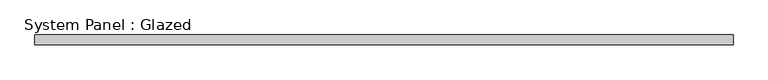
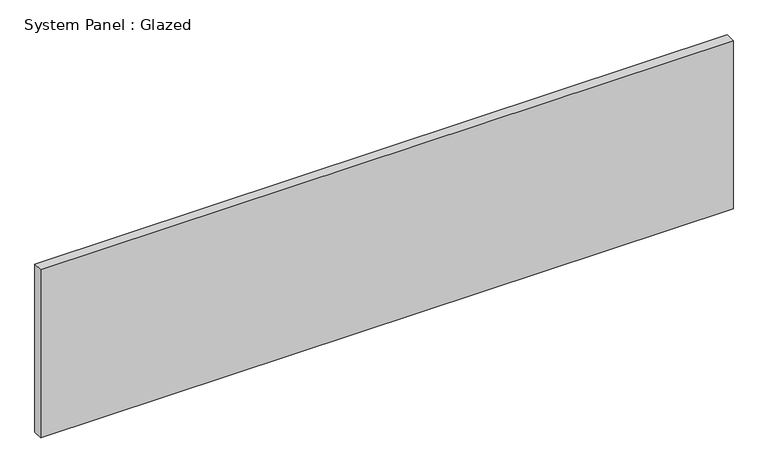
"""IFC4 building model written with IfcOpenShell, lengths in millimetres: plate geometry, System Panel : Glazed."""

import ifcopenshell
import ifcopenshell.guid

model = None  # the IFC model being written
_history = None  # IfcOwnerHistory: only IFC2X3 demands one
_inside = {}  # id of a spatial element -> (the spatial element, [elements in it])
_under = {}  # id of a project, library or spatial element -> (it, [spatial elements below it])
_declared = {}  # id of a project -> (the project, [libraries it declares])
_typed = {}  # id of a type object -> (the type object, [elements of that type])
_made_of = {}  # id of a material, layer set ... -> (it, [elements and type objects made of it])


def new_model(schema):
    """Start an empty IFC model of exactly this schema.

    Asked for "IFC4X3", IfcOpenShell would pick the latest addendum, in which some entities
    have other attributes; the version numbers below select the first issue.
    IFC2X3 requires an IfcOwnerHistory on every rooted entity: one is made here for all.
    """
    global model, _history
    if schema == "IFC4X3":
        model = ifcopenshell.file(schema_version=(4, 3, 0, 0))
    else:
        model = ifcopenshell.file(schema=schema)
    _inside.clear()
    _under.clear()
    _declared.clear()
    _typed.clear()
    _made_of.clear()
    _history = None
    if model.schema == "IFC2X3":
        org = make("IfcOrganization", Name="unknown")
        user = make(
            "IfcPersonAndOrganization",
            ThePerson=make("IfcPerson", FamilyName="unknown"),
            TheOrganization=org,
        )
        app = make(
            "IfcApplication",
            ApplicationDeveloper=org,
            Version="unknown",
            ApplicationFullName="unknown",
            ApplicationIdentifier="unknown",
        )
        _history = make(
            "IfcOwnerHistory",
            OwningUser=user,
            OwningApplication=app,
            ChangeAction="ADDED",
            CreationDate=0,
        )
    return model


def make(cls, **values):
    """One entity of the class cls with the attributes given. An attribute that is None is left unset."""
    return model.create_entity(
        cls, **{name: value for name, value in values.items() if value is not None}
    )


def rooted(cls, **values):
    """An entity with a GlobalId (a new one), such as an element, a storey or a relation."""
    return make(cls, GlobalId=ifcopenshell.guid.new(), OwnerHistory=_history, **values)


def si_unit(unit_type, name, prefix=None):
    """IfcSIUnit, for example si_unit("LENGTHUNIT", "METRE", prefix="MILLI")."""
    return make("IfcSIUnit", UnitType=unit_type, Prefix=prefix, Name=name)


def assignment(units):
    """IfcUnitAssignment: the units of a project."""
    return None if units is None else make("IfcUnitAssignment", Units=units)


def point(xyz):
    """IfcCartesianPoint."""
    return None if xyz is None else make("IfcCartesianPoint", Coordinates=xyz)


def direction(xyz):
    """IfcDirection."""
    return None if xyz is None else make("IfcDirection", DirectionRatios=xyz)


def frame(location, z_axis=None, x_axis=None):
    """IfcAxis2Placement3D, a coordinate frame: its origin and axes. An axis left out is left unset."""
    return make(
        "IfcAxis2Placement3D",
        Location=point(location),
        Axis=direction(z_axis),
        RefDirection=direction(x_axis),
    )


def origin():
    """The frame at (0, 0, 0) with its axes left unset."""
    return frame((0.0, 0.0, 0.0))


def origin_with_axes():
    """The frame at (0, 0, 0) with the z axis (0, 0, 1) and the x axis (1, 0, 0) written out."""
    return frame((0.0, 0.0, 0.0), z_axis=(0.0, 0.0, 1.0), x_axis=(1.0, 0.0, 0.0))


def place(relative_to, where):
    """IfcLocalPlacement: puts the frame where relative to a parent placement (None: the world)."""
    return make(
        "IfcLocalPlacement", PlacementRelTo=relative_to, RelativePlacement=where
    )


def context(
    kind, dimensions, precision=None, world=None, true_north=None, identifier=None
):
    """IfcGeometricRepresentationContext, for example the 3D "Model" context."""
    return make(
        "IfcGeometricRepresentationContext",
        ContextIdentifier=identifier,
        ContextType=kind,
        CoordinateSpaceDimension=dimensions,
        Precision=precision,
        WorldCoordinateSystem=world,
        TrueNorth=true_north,
    )


def project(units=None, contexts=None):
    """IfcProject with its units and contexts."""
    return rooted(
        "IfcProject",
        Name="project",
        RepresentationContexts=contexts,
        UnitsInContext=assignment(units),
    )


def spatial(cls, under=None, at=None, **own):
    """A site, building, storey or space (cls), placed at a placement, below another one or the project."""
    s = rooted(cls, ObjectPlacement=at, **own)
    if under is not None:
        _under.setdefault(under.id(), (under, []))[1].append(s)
    return s


def polyline(points):
    """IfcPolyline through the points."""
    return make("IfcPolyline", Points=[point(p) for p in points])


def outline(outer, holes=None, kind="AREA"):
    """IfcArbitraryClosedProfileDef: a profile drawn as a closed curve; with holes, ...WithVoids."""
    if holes is None:
        return make("IfcArbitraryClosedProfileDef", ProfileType=kind, OuterCurve=outer)
    return make(
        "IfcArbitraryProfileDefWithVoids",
        ProfileType=kind,
        OuterCurve=outer,
        InnerCurves=holes,
    )


def extrude(swept, where, along, depth):
    """IfcExtrudedAreaSolid: the profile swept, set in the frame where, extruded along a direction by depth."""
    return make(
        "IfcExtrudedAreaSolid",
        SweptArea=swept,
        Position=where,
        ExtrudedDirection=direction(along),
        Depth=depth,
    )


def shape(context_of_items, identifier, shape_type, items):
    """IfcShapeRepresentation: the items that make up one representation, for example the "Body"."""
    return make(
        "IfcShapeRepresentation",
        ContextOfItems=context_of_items,
        RepresentationIdentifier=identifier,
        RepresentationType=shape_type,
        Items=items,
    )


def source(mapping_origin, context_of_items, identifier, shape_type, items):
    """IfcRepresentationMap: a shape defined once, which mapped items show again and again."""
    return make(
        "IfcRepresentationMap",
        MappingOrigin=mapping_origin,
        MappedRepresentation=shape(context_of_items, identifier, shape_type, items),
    )


def transform(
    local_origin,
    x_axis=None,
    y_axis=None,
    z_axis=None,
    scale=None,
    scale2=None,
    scale3=None,
    uniform=True,
):
    """IfcCartesianTransformationOperator3D, or its non-uniform kind. x_axis, y_axis, z_axis: its Axis1, 2, 3."""
    if uniform:
        return make(
            "IfcCartesianTransformationOperator3D",
            Axis1=direction(x_axis),
            Axis2=direction(y_axis),
            LocalOrigin=point(local_origin),
            Scale=scale,
            Axis3=direction(z_axis),
        )
    return make(
        "IfcCartesianTransformationOperator3DnonUniform",
        Axis1=direction(x_axis),
        Axis2=direction(y_axis),
        LocalOrigin=point(local_origin),
        Scale=scale,
        Axis3=direction(z_axis),
        Scale2=scale2,
        Scale3=scale3,
    )


def mapped(mapping_source, mapping_target):
    """IfcMappedItem: shows the shape of a source again, moved by a transform."""
    return make(
        "IfcMappedItem", MappingSource=mapping_source, MappingTarget=mapping_target
    )


def made_of(thing, what):
    """Note that an element or type object is made of a material, layer set ...; save() writes the relation."""
    if what is not None:
        _made_of.setdefault(what.id(), (what, []))[1].append(thing)
    return thing


def element(
    cls,
    number,
    at=None,
    inside=None,
    cuts=None,
    type_object=None,
    material=None,
    context=None,
    identifier="Body",
    shape_type=None,
    held_by="IfcProductDefinitionShape",
    body=None,
    shapes=None,
    **own,
):
    """One element of the class cls, such as IfcWall. Its Tag is "e" and its number.

    at: its placement. inside: the storey or other place that contains it. cuts: it is an
    opening in that element (IfcRelVoidsElement). A single representation is given by context,
    identifier, shape_type and body (its items); several are given by shapes. held_by: the class
    of the entity that holds the representations. save() writes the other relations.
    """
    e = rooted(cls, Tag="e%d" % number, ObjectPlacement=at, **own)
    if body is not None:
        shapes = [shape(context, identifier, shape_type, body)]
    if shapes is not None:
        e.Representation = make(held_by, Representations=shapes)
    if inside is not None:
        _inside.setdefault(inside.id(), (inside, []))[1].append(e)
    if cuts is not None:
        rooted(
            "IfcRelVoidsElement", RelatingBuildingElement=cuts, RelatedOpeningElement=e
        )
    if type_object is not None:
        _typed.setdefault(type_object.id(), (type_object, []))[1].append(e)
    return made_of(e, material)


def aggregate(whole, parts):
    """IfcRelAggregates: a whole, such as a stair, and the parts it consists of."""
    return rooted("IfcRelAggregates", RelatingObject=whole, RelatedObjects=parts)


def save(model, path):
    """Write the relations noted so far, then the file.

    IfcRelAggregates (storeys below a building ...), IfcRelContainedInSpatialStructure (elements
    in a storey), IfcRelDefinesByType, IfcRelAssociatesMaterial and IfcRelDeclares: one each for
    every whole, place, type object, material and project.
    """
    for whole, parts in _under.values():
        aggregate(whole, parts)
    for where, things in _inside.values():
        rooted(
            "IfcRelContainedInSpatialStructure",
            RelatedElements=things,
            RelatingStructure=where,
        )
    for kind, things in _typed.values():
        rooted("IfcRelDefinesByType", RelatedObjects=things, RelatingType=kind)
    for what, things in _made_of.values():
        rooted("IfcRelAssociatesMaterial", RelatedObjects=things, RelatingMaterial=what)
    for by, libraries in _declared.values():
        rooted("IfcRelDeclares", RelatingContext=by, RelatedDefinitions=libraries)
    model.write(path)


def system_panel_glazed_bd903948(model_context):
    return source(origin(), model_context, "Body", "SweptSolid", [
        extrude(outline(polyline([(877.5, -49.5), (-877.5, -49.5), (-877.5, -24.5), (877.5, -24.5), (877.5, -49.5)])), origin_with_axes(), (0.0, 0.0, 1.0), 450.0),
    ])


if __name__ == "__main__":
    model = new_model("IFC4")
    model_context = context("Model", 3, world=origin())
    ifc_project = project(units=[si_unit("LENGTHUNIT", "METRE", prefix="MILLI")], contexts=[model_context])
    site = spatial("IfcSite", under=ifc_project)
    building = spatial("IfcBuilding", under=site)
    placement = place(None, origin())
    system_panel_glazed_shape = system_panel_glazed_bd903948(model_context)
    element("IfcPlate", 1, ObjectType="System Panel : Glazed", at=placement, inside=building, context=model_context, shape_type="MappedRepresentation", body=[
        mapped(system_panel_glazed_shape, transform((0.0, 0.0, 0.0), x_axis=(1.0, 0.0, 0.0), y_axis=(0.0, 1.0, 0.0), z_axis=(0.0, 0.0, 1.0))),
    ])
    save(model, "model.ifc")

# Revit data of these elements
# Type "System Panel : Glazed"
#   Keynote = "H11"
#   Construction Type Id = "GSP4R"
#   Analytic Construction = "1/8 in Pilkington single glazing"
#   Visual Light Transmittance = 0.9
#   Solar Heat Gain Coefficient = 0.86
#   Heat Transfer Coefficient (U) = 6.7069 W/(m²·K)
# Element 1 (IfcPlate, "System Panel : Glazed")
#   Materials on its faces: "Glass"
# Materials
#   "Glass": class "Glass", colour RGB 0 128 192, transparency 0.9, Description = "Soda Lime Glass", Cost = 0
